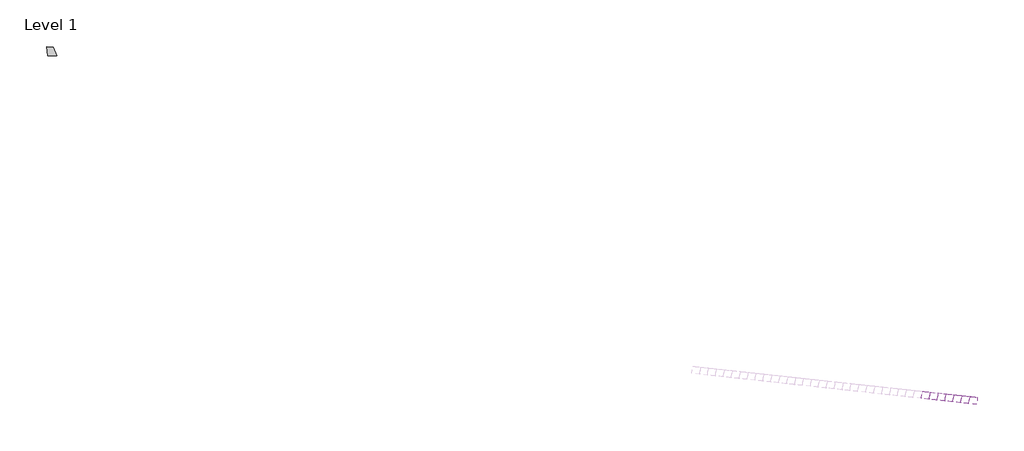
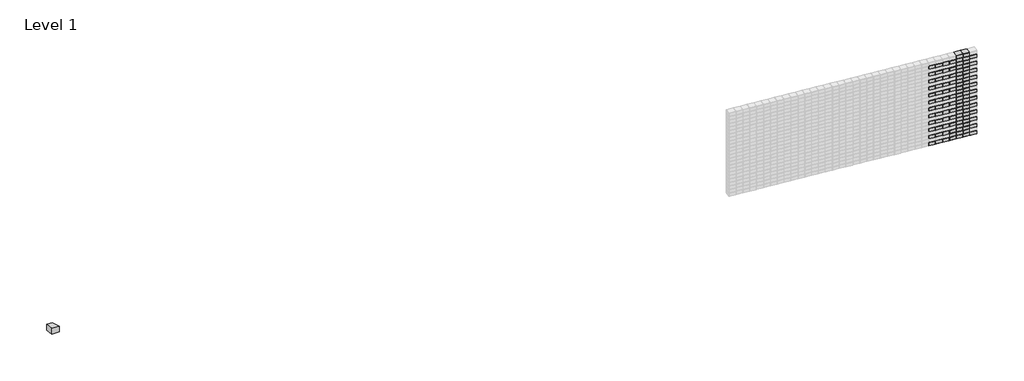
# One storey, part 18 of 18: 111 proxies.
# Revit data of these elements (continued)
# Elements 1, 2, 3, 4, 5, 6, 7, 8, 9, 10, 11, 12, 13 (IfcBuildingElementProxy, "00_GMA_steen_versie_6 : Geel") (continued)
#   StootvoegLinksHalfBoven = 0 mm
#   StootVoegRechtsHalfOnder = 5 mm
#   StootVoegRechtsHalfBoven = 5 mm
#   StootVoegBreedteRechts = 10 mm
#   StootVoegBreedteLinks = 0 mm
#   LintVoegOnderHalf = 5 mm
#   LintVoegOnder = 10 mm
#   LintVoegBovenHalf = 5 mm
#   LintVoegBoven = 10 mm
#   Phase Created = New Construction
#   Materials on its faces: "20_voeg", "21_steen_geel"
# Elements 14, 15, 16, 17, 18, 19, 20, 21, 22, 23, 24, 25 (IfcBuildingElementProxy, "00_GMA_steen_versie_6 : Geel")
#   StootvoegLinksHalfOnder = 5 mm
#   StootvoegLinksHalfBoven = 5 mm
#   StootVoegRechtsHalfOnder = 0 mm
#   StootVoegRechtsHalfBoven = 0 mm
#   StootVoegBreedteRechts = 0 mm
#   StootVoegBreedteLinks = 10 mm
#   LintVoegOnderHalf = 5 mm
#   LintVoegOnder = 10 mm
#   LintVoegBovenHalf = 5 mm
#   LintVoegBoven = 10 mm
#   Phase Created = New Construction
#   Materials on its faces: "20_voeg", "21_steen_geel"
# Elements 26, 27, 28, 29, 30, 31, 32, 33, 34, 35, 36, 37 (IfcBuildingElementProxy, "00_GMA_steen_versie_6 : Rood")
#   StootvoegLinksHalfOnder = 0 mm
#   StootvoegLinksHalfBoven = 0 mm
#   StootVoegRechtsHalfOnder = 5 mm
#   StootVoegRechtsHalfBoven = 5 mm
#   StootVoegBreedteRechts = 10 mm
#   StootVoegBreedteLinks = 0 mm
#   LintVoegOnderHalf = 5 mm
#   LintVoegOnder = 10 mm
#   LintVoegBovenHalf = 5 mm
#   LintVoegBoven = 10 mm
#   Phase Created = New Construction
#   Materials on its faces: "20_voeg", "21_steen_rood"
# Elements 38, 39, 40, 41, 42, 43, 44, 45, 46, 47, 48, 49, 50, 51, 52, 53, 54, 55, 56, 57, 58, 59, 60, 61, 62, 63, 64, 65, 66, 67, 68, 69, 70, 71, 72, 73, 74, 75, 76, 77, 78, 79, 80, 81, 82, 83, 84, 85, 86, 87, 88, 89, 90, 91, 92, 93, 94, 95, 96, 97 (IfcBuildingElementProxy, "00_GMA_steen_versie_6 : Rood")
#   StootvoegLinksHalfOnder = 5 mm
#   StootvoegLinksHalfBoven = 5 mm
#   StootVoegRechtsHalfOnder = 5 mm
#   StootVoegRechtsHalfBoven = 5 mm
#   StootVoegBreedteRechts = 10 mm
#   StootVoegBreedteLinks = 10 mm
#   LintVoegOnderHalf = 5 mm
#   LintVoegOnder = 10 mm
#   LintVoegBovenHalf = 5 mm
#   LintVoegBoven = 10 mm
#   Phase Created = New Construction
#   Materials on its faces: "20_voeg", "21_steen_rood"
# Elements 98, 99, 100, 101, 102, 103, 104, 105, 106, 107, 108, 109 (IfcBuildingElementProxy, "00_GMA_steen_versie_6 : Rood")
#   StootvoegLinksHalfOnder = 5 mm
#   StootvoegLinksHalfBoven = 5 mm
#   StootVoegRechtsHalfOnder = 5 mm
#   StootVoegRechtsHalfBoven = 5 mm
#   StootVoegBreedteRechts = 10 mm
#   StootVoegBreedteLinks = 10 mm
#   LintVoegOnderHalf = 0 mm
#   LintVoegOnder = 0 mm
#   LintVoegBovenHalf = 5 mm
#   LintVoegBoven = 10 mm
#   Phase Created = New Construction
#   Materials on its faces: "20_voeg", "21_steen_rood"
# Element 110 (IfcBuildingElementProxy, "00_GMA_steen_versie_5 : Steen Geel")
#   StootVoegHalfBoven = 5 mm
#   StootVoegHalf = 5 mm
#   Phase Created = New Construction
#   Materials on its faces: "21_steen_geel"
# Element 111 (IfcBuildingElementProxy, "00_GMA_steen_versie_4 : Steen Standaard Rood")
#   StootVoegHalfBoven = 5 mm
#   StootVoegHalf = 5 mm
#   Phase Created = New Construction
#   Materials on its faces: "21_steen_rood"
# Materials
#   "21_steen_geel": class "Unassigned", colour RGB 202 202 0, transparency 0, Cost = 0
#   "20_voeg": class "Concrete", colour RGB 86 86 86, transparency 0, Manufacturer = "RevitGG", URL = "www.revitgg.nl", Description = "zandcement, generiek materiaal", Cost = 0
#   "21_steen_rood": class "Unassigned", colour RGB 213 111 43, transparency 0, Cost = 0
